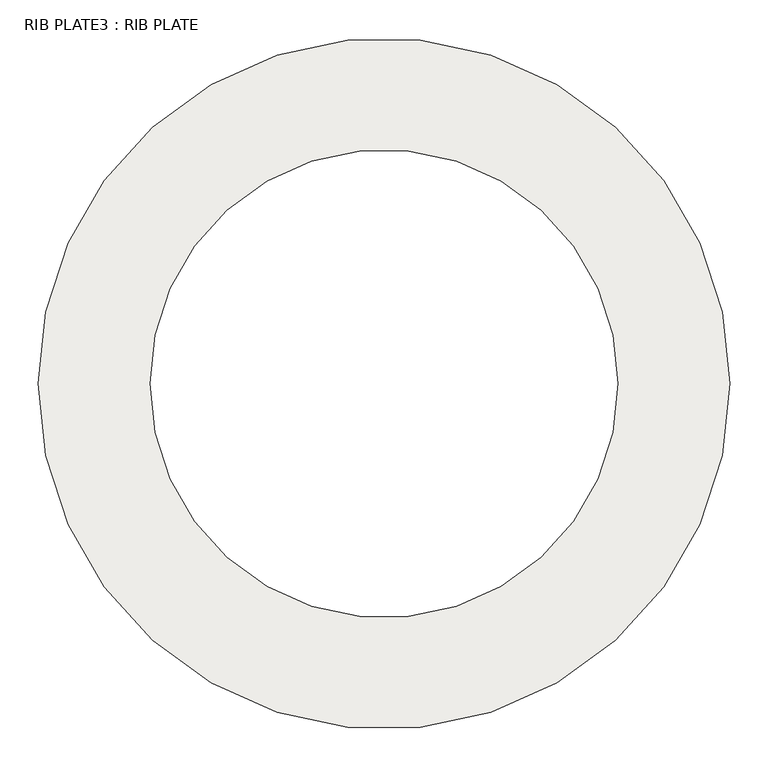
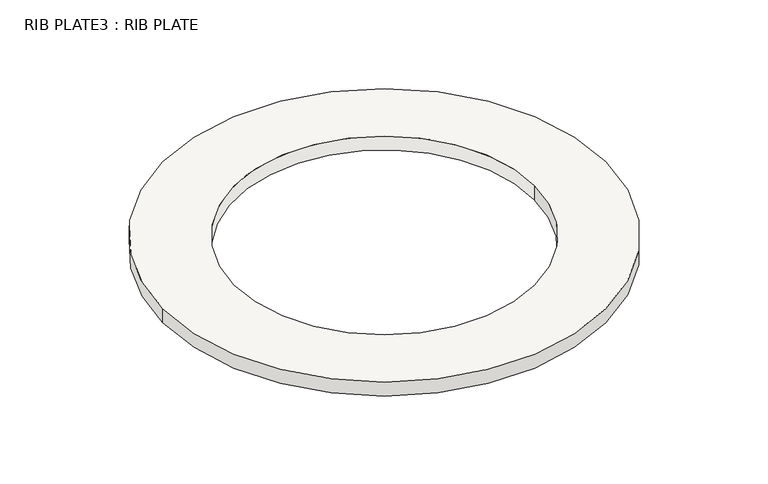
"""IFC4 building model written with IfcOpenShell, lengths in millimetres: slab geometry, RIB PLATE3 : RIB PLATE."""

from ifc_helpers import new_model, si_unit, point, frame, frame_2d, origin, place, context, project, spatial, circle_curve, trimmed, segment, composite_curve, outline, extrude, source, transform, mapped, element, save


def rib_plate3_rib_plate_2686f07b(model_context):
    return source(origin(), model_context, "Body", "SweptSolid", [
        extrude(outline(composite_curve([segment(trimmed(circle_curve(frame_2d((7920.0, 66679.5208589)), 450.0), [point((7470.0, 66679.5208589))], [point((8370.0, 66679.5208589))], False, "CARTESIAN"), True, "CONTINUOUS"), segment(trimmed(circle_curve(frame_2d((7920.0, 66679.5208589)), 450.0), [point((8370.0, 66679.5208589))], [point((7470.0, 66679.5208589))], False, "CARTESIAN"), True, "CONTINUOUS")], self_intersect=False), holes=[composite_curve([segment(trimmed(circle_curve(frame_2d((7920.0, 66679.5208589)), 304.6641594), [point((7615.3358406, 66679.5208589))], [point((8224.6641594, 66679.5208589))], True, "CARTESIAN"), True, "CONTINUOUS"), segment(trimmed(circle_curve(frame_2d((7920.0, 66679.5208589)), 304.6641594), [point((8224.6641594, 66679.5208589))], [point((7615.3358406, 66679.5208589))], True, "CARTESIAN"), True, "CONTINUOUS")], self_intersect=False)]), frame((0.0, 0.0, -1030.0), z_axis=(0.0, 0.0, 1.0), x_axis=(1.0, 0.0, 0.0)), (0.0, 0.0, 1.0), 30.0),
    ])


if __name__ == "__main__":
    model = new_model("IFC4")
    model_context = context("Model", 3, world=origin())
    ifc_project = project(units=[si_unit("LENGTHUNIT", "METRE", prefix="MILLI")], contexts=[model_context])
    site = spatial("IfcSite", under=ifc_project)
    building = spatial("IfcBuilding", under=site)
    placement = place(None, origin())
    rib_plate3_rib_plate_shape = rib_plate3_rib_plate_2686f07b(model_context)
    element("IfcSlab", 1, ObjectType="RIB PLATE3 : RIB PLATE", at=placement, inside=building, context=model_context, shape_type="MappedRepresentation", body=[
        mapped(rib_plate3_rib_plate_shape, transform((0.0, 0.0, 0.0), x_axis=(1.0, 0.0, 0.0), y_axis=(0.0, 1.0, 0.0), z_axis=(0.0, 0.0, 1.0))),
    ])
    save(model, "model.ifc")

# Revit data of these elements
# Element 1 (IfcSlab, "RIB PLATE3 : RIB PLATE")
#   Materials on its faces: "Metal - Steel"
# Materials
#   "Metal - Steel": class "Metal", colour RGB 247 247 247, transparency 0, Cost = 0
